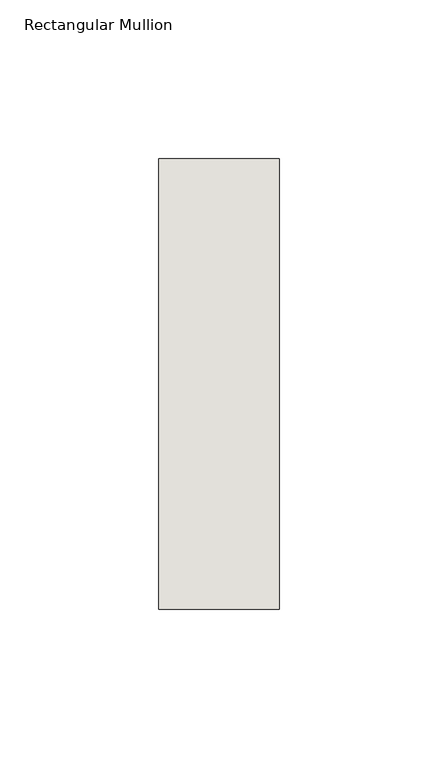
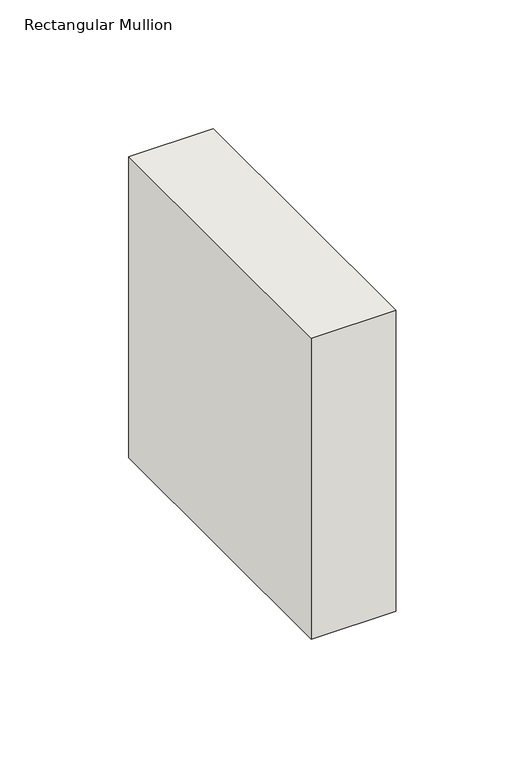
"""IFC4 building model written with IfcOpenShell, lengths in millimetres: wall geometry, Rectangular Mullion : NLRS_21_CWM_hsb-regel 38x142_gen_rsf."""

from ifc_helpers import new_model, si_unit, frame, origin, place, context, project, spatial, polyline, outline, extrude, source, transform, mapped, element, save


def rectangular_mullion_f3eb0596(model_context):
    return source(origin(), model_context, "Body", "SweptSolid", [
        extrude(outline(polyline([(0.0, -71.0), (-38.0, -71.0), (-38.0, 71.0), (0.0, 71.0), (0.0, -71.0)])), frame((0.0, 0.0, -142.9999997), z_axis=(0.0, 0.0, 1.0), x_axis=(1.0, 0.0, 0.0)), (0.0, 0.0, 1.0), 142.9999997),
    ])


if __name__ == "__main__":
    model = new_model("IFC4")
    model_context = context("Model", 3, world=origin())
    ifc_project = project(units=[si_unit("LENGTHUNIT", "METRE", prefix="MILLI")], contexts=[model_context])
    site = spatial("IfcSite", under=ifc_project)
    building = spatial("IfcBuilding", under=site)
    placement = place(None, origin())
    rectangular_mullion_shape = rectangular_mullion_f3eb0596(model_context)
    element("IfcWall", 1, ObjectType="Rectangular Mullion : NLRS_21_CWM_hsb-regel 38x142_gen_rsf", at=placement, inside=building, context=model_context, shape_type="MappedRepresentation", body=[
        mapped(rectangular_mullion_shape, transform((0.0, 0.0, 0.0), x_axis=(1.0, 0.0, 0.0), y_axis=(0.0, 1.0, 0.0), z_axis=(0.0, 0.0, 1.0))),
    ])
    save(model, "model.ifc")

# Revit data of these elements
# Type "Rectangular Mullion : NLRS_21_CWM_hsb-regel 38x142_gen_rsf"
#   Type IfcGUID = "07M7mRoiH1CR8m_RSKIwpF"
#   Assembly Code = "21.10"
#   IfcExportAs = "IfcWall"
#   built-in parameter 1007322 = 0.465879 (stored number, unit not read)
#   built-in parameter 1007321 = 0.062336 (stored number, unit not read)
#   built-in parameter 1007320 = 0.062336 (stored number, unit not read)
# Element 1 (IfcWall, "Rectangular Mullion : NLRS_21_CWM_hsb-regel 38x142_gen_rsf")
#   Materials on its faces: "NLRS_i2_hout naaldhout vuren_gen_rsf"
# Materials
#   "NLRS_i2_hout naaldhout vuren_gen_rsf": class "I - Hout", colour RGB 234 199 147, transparency 0, Keynote = "i2", Manufacturer = "Revit Standards Foundation", URL = "www.revitstandards.org", Description = "hout vuren", Cost = 0
